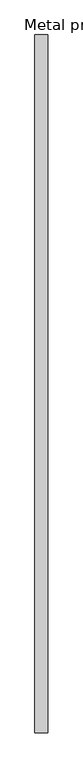
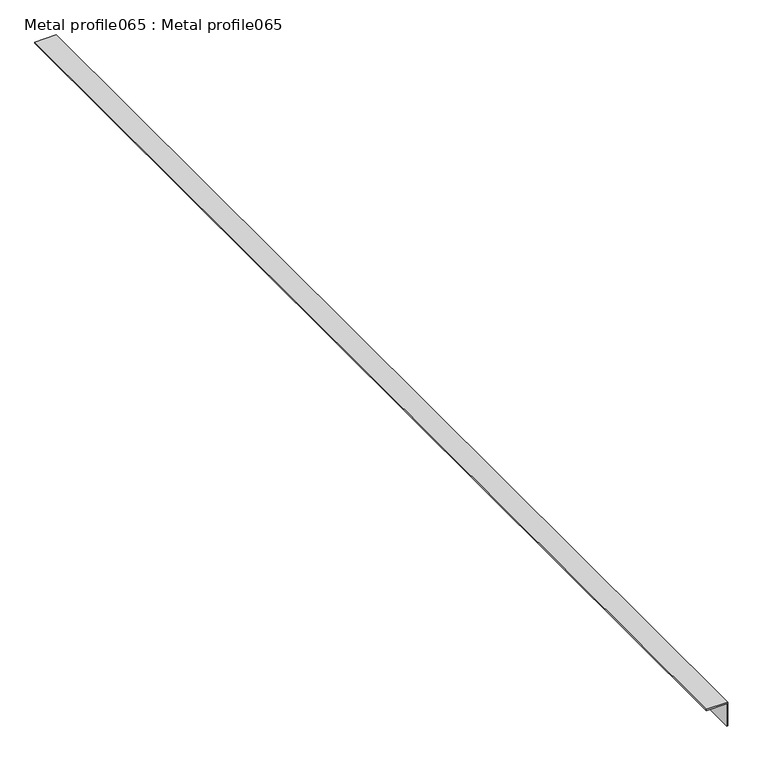
"""IFC4 building model written with IfcOpenShell, lengths in millimetres: proxy geometry, Metal profile065 : Metal profile065."""

from ifc_helpers import new_model, si_unit, frame, origin, place, context, project, spatial, polyline, outline, extrude, source, transform, mapped, element, save


def metal_profile065_metal_profile065_504d0bb8(model_context):
    return source(origin(), model_context, "Body", "SweptSolid", [
        extrude(outline(polyline([(36399.8671875, -6102.5366211), (36399.8671875, -6067.5405273), (36358.9765625, -6067.5405273), (36358.9765625, -6065.5405273), (36401.8671875, -6065.5405273), (36401.8671875, -6102.5366211), (36399.8671875, -6102.5366211)])), frame((0.0, -1052.8906574, 0.0), z_axis=(0.0, 1.0, 0.0), x_axis=(0.0, 0.0, 1.0)), (0.0, 0.0, 1.0), 2000.0),
    ])


if __name__ == "__main__":
    model = new_model("IFC4")
    model_context = context("Model", 3, world=origin())
    ifc_project = project(units=[si_unit("LENGTHUNIT", "METRE", prefix="MILLI")], contexts=[model_context])
    site = spatial("IfcSite", under=ifc_project)
    building = spatial("IfcBuilding", under=site)
    placement = place(None, origin())
    metal_profile065_metal_profile065_shape = metal_profile065_metal_profile065_504d0bb8(model_context)
    element("IfcBuildingElementProxy", 1, Name="Metal profile065 : Metal profile065", ObjectType="Metal profile065 : Metal profile065", at=placement, inside=building, context=model_context, shape_type="MappedRepresentation", body=[
        mapped(metal_profile065_metal_profile065_shape, transform((0.0, 0.0, 0.0), x_axis=(1.0, 0.0, 0.0), y_axis=(0.0, 1.0, 0.0), z_axis=(0.0, 0.0, 1.0))),
    ])
    save(model, "model.ifc")

# Revit data of these elements
# Type "Metal profile065 : Metal profile065"
#   NameOverride = "Metal profile065"
# Element 1 (IfcBuildingElementProxy, "Metal profile065 : Metal profile065")
#   Materials on its faces: "L-SHAPED METAL TRIM"
# Materials
#   "L-SHAPED METAL TRIM": class "Unassigned", colour RGB 255 231 0, transparency 0
